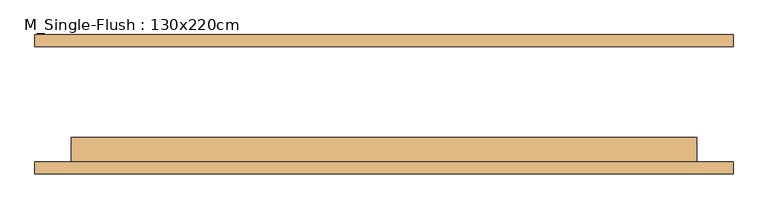
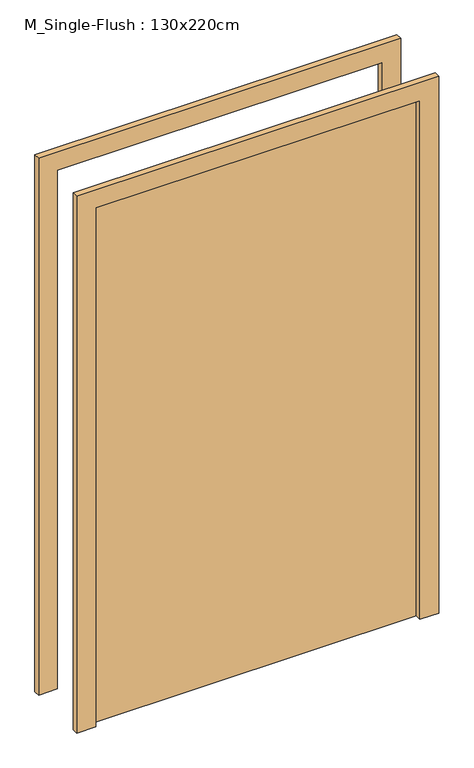
"""IFC4 building model written with IfcOpenShell, lengths in millimetres: door geometry, M_Single-Flush : 130x220cm."""

from ifc_helpers import new_model, si_unit, frame, origin, origin_with_axes, place, context, project, spatial, polyline, outline, extrude, source, transform, mapped, element, save


def m_single_flush_130x220cm_99d74091(model_context):
    return source(origin(), model_context, "Body", "SweptSolid", [
        extrude(outline(polyline([(2276.0, -726.0), (0.0, -726.0), (0.0, -650.0), (2200.0, -650.0), (2200.0, 650.0), (0.0, 650.0), (0.0, 726.0), (2276.0, 726.0), (2276.0, -726.0)])), frame((0.0, -145.0, 0.0), z_axis=(0.0, 1.0, 0.0), x_axis=(0.0, 0.0, 1.0)), (0.0, 0.0, 1.0), 25.0),
        extrude(outline(polyline([(2276.0, 726.0), (2276.0, -726.0), (0.0, -726.0), (0.0, -650.0), (2200.0, -650.0), (2200.0, 650.0), (0.0, 650.0), (0.0, 726.0), (2276.0, 726.0)])), frame((0.0, 120.0, 0.0), z_axis=(0.0, 1.0, 0.0), x_axis=(0.0, 0.0, 1.0)), (0.0, 0.0, 1.0), 25.0),
        extrude(outline(polyline([(650.0, -69.0), (650.0, -120.0), (-650.0, -120.0), (-650.0, -69.0), (650.0, -69.0)])), origin_with_axes(), (0.0, 0.0, 1.0), 2200.0),
    ])


if __name__ == "__main__":
    model = new_model("IFC4")
    model_context = context("Model", 3, world=origin())
    ifc_project = project(units=[si_unit("LENGTHUNIT", "METRE", prefix="MILLI")], contexts=[model_context])
    site = spatial("IfcSite", under=ifc_project)
    building = spatial("IfcBuilding", under=site)
    placement = place(None, origin())
    m_single_flush_130x220cm_shape = m_single_flush_130x220cm_99d74091(model_context)
    element("IfcDoor", 1, ObjectType="M_Single-Flush : 130x220cm", at=placement, inside=building, context=model_context, shape_type="MappedRepresentation", body=[
        mapped(m_single_flush_130x220cm_shape, transform((0.0, 0.0, 0.0), x_axis=(1.0, 0.0, 0.0), y_axis=(0.0, 1.0, 0.0), z_axis=(0.0, 0.0, 1.0))),
    ])
    save(model, "model.ifc")

# Revit data of these elements
# Type "M_Single-Flush : 130x220cm"
#   Type Mark = "46"
#   Construction Type Id = "MDOOR"
#   Analytic Construction = "Metal"
#   Thickness = 5.10 cm
#   Heat Transfer Coefficient (U) = 3.7021 W/(m²·K)
#   Height = 220.00 cm
#   Trim Projection Ext = 2.50 cm
#   Trim Projection Int = 2.50 cm
#   Trim Width = 7.60 cm
#   Width = 130.00 cm
#   Define Thermal Properties by = 1
#   Door Material = Door - Panel
#   Frame Material = Door - Frame
#   Visual Light Transmittance = 0
#   Solar Heat Gain Coefficient = 0
#   Function = (empty or 0)
#   Wall Closure = (empty or 0)
# Element 1 (IfcDoor, "M_Single-Flush : 130x220cm")
#   Materials on its faces: "Door - Frame", "Door - Panel"
# Materials
#   "Door - Panel": class "Wood", colour RGB 210 159 95, transparency 0, Cost = 0
#   "Door - Frame": class "Miscellaneous", colour RGB 118 70 51, transparency 0, Cost = 0
